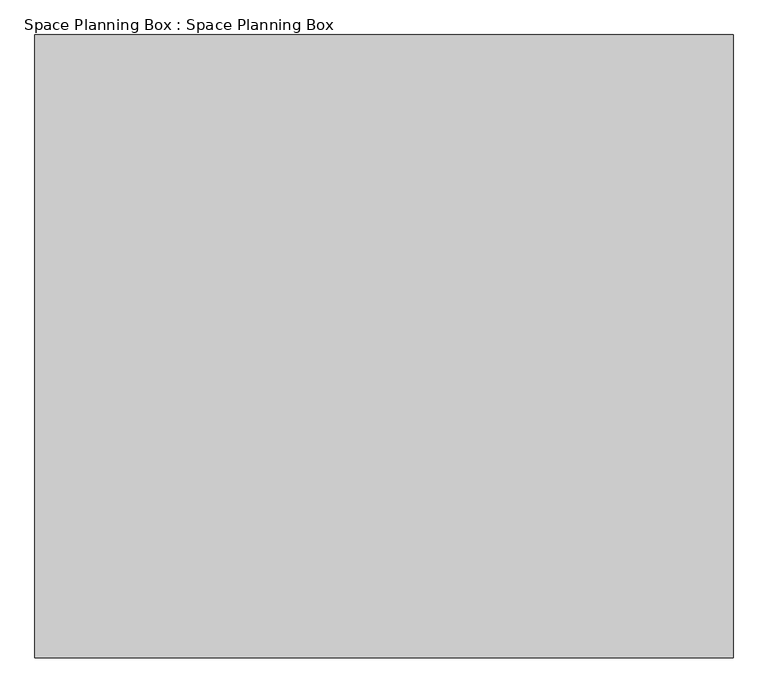
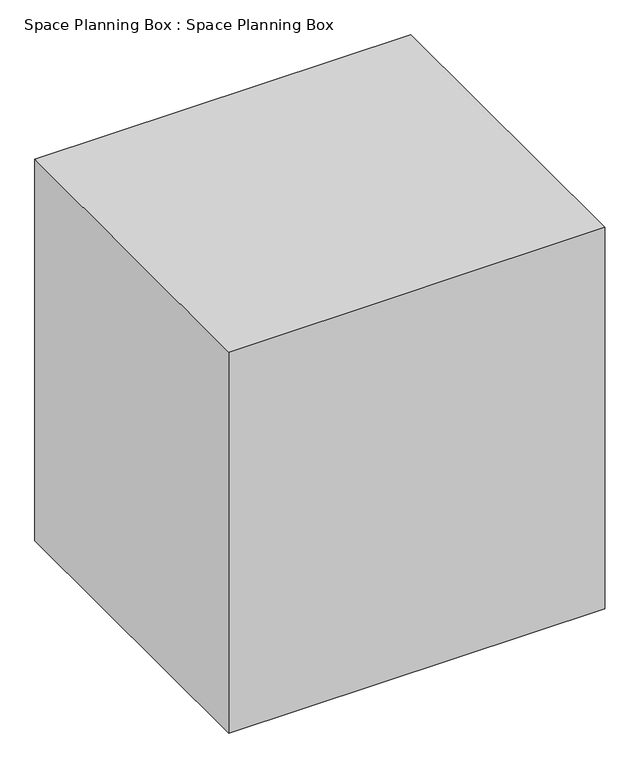
"""IFC4 building model written with IfcOpenShell, lengths in millimetres: proxy geometry, Space Planning Box : Space Planning Box."""

from ifc_helpers import new_model, si_unit, origin, origin_with_axes, place, context, project, spatial, polyline, outline, extrude, source, transform, mapped, element, save


def space_planning_box_space_planning_box_c1734578(model_context):
    return source(origin(), model_context, "Body", "SweptSolid", [
        extrude(outline(polyline([(2800.0, 2500.0), (2800.0, -2500.0), (-2800.0, -2500.0), (-2800.0, 2500.0), (2800.0, 2500.0)])), origin_with_axes(), (0.0, 0.0, 1.0), 6000.0),
    ])


if __name__ == "__main__":
    model = new_model("IFC4")
    model_context = context("Model", 3, world=origin())
    ifc_project = project(units=[si_unit("LENGTHUNIT", "METRE", prefix="MILLI")], contexts=[model_context])
    site = spatial("IfcSite", under=ifc_project)
    building = spatial("IfcBuilding", under=site)
    placement = place(None, origin())
    space_planning_box_space_planning_box_shape = space_planning_box_space_planning_box_c1734578(model_context)
    element("IfcBuildingElementProxy", 1, Name="Space Planning Box : Space Planning Box", ObjectType="Space Planning Box : Space Planning Box", at=placement, inside=building, context=model_context, shape_type="MappedRepresentation", body=[
        mapped(space_planning_box_space_planning_box_shape, transform((0.0, 0.0, 0.0), x_axis=(1.0, 0.0, 0.0), y_axis=(0.0, 1.0, 0.0), z_axis=(0.0, 0.0, 1.0))),
    ])
    save(model, "model.ifc")

# Revit data of these elements
# Type "Space Planning Box : Space Planning Box"
#   Type Comments = "..."
#   Room Name [instance default] = "?"
#   Assembly Code = "..."
#   Width [instance default] = 1524 mm
#   Program Area [instance default] = 0 m²
#   Length [instance default] = 1524 mm
#   Height [instance default] = 1524 mm
#   Area [instance default] = 2.32258 m²
#   Fill Color [instance default] = Cyan
#   Default Elevation = 0
# Element 1 (IfcBuildingElementProxy, "Space Planning Box : Space Planning Box")
#   Room Name = "Locker Room (M)"
#   Width = 5600 mm
#   Program Area = 31.5 m²
#   Length = 5000 mm
#   Height = 6000 mm
#   Area = 28 m²
#   Fill Color = Lavender
#   Materials on its faces: "Lavender"
# Materials
#   "Cyan": class "Generic", colour RGB 0 255 255, transparency 0.2, Cost = 0
#   "Lavender": class "Generic", colour RGB 186 85 211, transparency 0.2, Cost = 0
